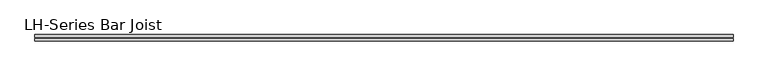
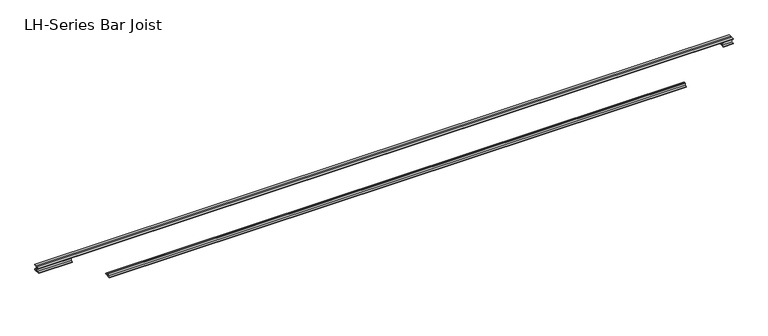
"""IFC4 building model written with IfcOpenShell, lengths in millimetres: beam geometry, LH-Series Bar Joist : 32LH-SP5."""

from ifc_helpers import new_model, si_unit, frame, origin, place, context, project, spatial, polyline, outline, extrude, source, transform, mapped, element, save


def lh_series_bar_joist_ab931e5b(model_context):
    return source(origin(), model_context, "Body", "SweptSolid", [
        extrude(outline(polyline([(12.7, 406.4), (76.2, 406.4), (76.2, 393.7), (25.4, 393.7), (25.4, 342.9), (12.7, 342.9), (12.7, 406.4)])), frame((-8381.9219944, 0.0, 0.0), z_axis=(1.0, 0.0, 0.0), x_axis=(0.0, 1.0, 0.0)), (0.0, 0.0, 1.0), 16208.2969944),
        extrude(outline(polyline([(-12.7, 406.4), (-12.7, 342.9), (-25.4, 342.9), (-25.4, 393.7), (-76.2, 393.7), (-76.2, 406.4), (-12.7, 406.4)])), frame((-8381.9219944, 0.0, 0.0), z_axis=(1.0, 0.0, 0.0), x_axis=(0.0, 1.0, 0.0)), (0.0, 0.0, 1.0), 16208.2969944),
        extrude(outline(polyline([(12.7, -406.4), (12.7, -342.9), (25.4, -342.9), (25.4, -393.7), (76.2, -393.7), (76.2, -406.4), (12.7, -406.4)])), frame((-6734.175, 0.0, 0.0), z_axis=(1.0, 0.0, 0.0), x_axis=(0.0, 1.0, 0.0)), (0.0, 0.0, 1.0), 13468.35),
        extrude(outline(polyline([(-12.7, -406.4), (-76.2, -406.4), (-76.2, -393.7), (-25.4, -393.7), (-25.4, -342.9), (-12.7, -342.9), (-12.7, -406.4)])), frame((-6734.175, 0.0, 0.0), z_axis=(1.0, 0.0, 0.0), x_axis=(0.0, 1.0, 0.0)), (0.0, 0.0, 1.0), 13468.35),
        extrude(outline(polyline([(12.7, 279.4), (12.7, 342.9), (25.4, 342.9), (25.4, 292.1), (76.2, 292.1), (76.2, 279.4), (12.7, 279.4)])), frame((7597.775, 0.0, 0.0), z_axis=(1.0, 0.0, 0.0), x_axis=(0.0, 1.0, 0.0)), (0.0, 0.0, 1.0), 228.6),
        extrude(outline(polyline([(-12.7, 279.4), (-76.2, 279.4), (-76.2, 292.1), (-25.4, 292.1), (-25.4, 342.9), (-12.7, 342.9), (-12.7, 279.4)])), frame((7597.775, 0.0, 0.0), z_axis=(1.0, 0.0, 0.0), x_axis=(0.0, 1.0, 0.0)), (0.0, 0.0, 1.0), 228.6),
        extrude(outline(polyline([(-12.7, 279.4), (-76.2, 279.4), (-76.2, 292.1), (-25.4, 292.1), (-25.4, 342.9), (-12.7, 342.9), (-12.7, 279.4)])), frame((-8381.9219944, 0.0, 0.0), z_axis=(1.0, 0.0, 0.0), x_axis=(0.0, 1.0, 0.0)), (0.0, 0.0, 1.0), 784.1469944),
        extrude(outline(polyline([(76.2, 279.4), (12.7, 279.4), (12.7, 342.9), (25.4, 342.9), (25.4, 292.1), (76.2, 292.1), (76.2, 279.4)])), frame((-8381.9219944, 0.0, 0.0), z_axis=(1.0, 0.0, 0.0), x_axis=(0.0, 1.0, 0.0)), (0.0, 0.0, 1.0), 784.1469944),
    ])


if __name__ == "__main__":
    model = new_model("IFC4")
    model_context = context("Model", 3, world=origin())
    ifc_project = project(units=[si_unit("LENGTHUNIT", "METRE", prefix="MILLI")], contexts=[model_context])
    site = spatial("IfcSite", under=ifc_project)
    building = spatial("IfcBuilding", under=site)
    placement = place(None, origin())
    lh_series_bar_joist_shape = lh_series_bar_joist_ab931e5b(model_context)
    element("IfcBeam", 1, ObjectType="LH-Series Bar Joist : 32LH-SP5", at=placement, inside=building, context=model_context, shape_type="MappedRepresentation", body=[
        mapped(lh_series_bar_joist_shape, transform((0.0, 0.0, 0.0), x_axis=(1.0, 0.0, 0.0), y_axis=(0.0, 1.0, 0.0), z_axis=(0.0, 0.0, 1.0))),
    ])
    save(model, "model.ifc")

# Revit data of these elements
# Type "LH-Series Bar Joist : 32LH-SP5"
#   Assembly Code = "B1010350"
#   Wt = 30
#   Web Thickness = 0' - 1"
#   Variable Panel [instance default] = 5' - 4"
#   Start Offset [instance default] = 0' - 0"
#   Start Extension [instance default] = 0' - 0"
#   Seat Length = 0' - 6"
#   Seat Depth = 0' - 5"
#   IntPanelWidth [instance default] = 5' - 4"
#   IntPanelArrayLength [instance default] = 21' - 4"
#   PanelAreaLength [instance default] = 32' - 0"
#   End Panel = 4' - 0"
#   End Offset [instance default] = 0' - 0"
#   End Extension [instance default] = 0' - 0"
#   Cord Leg = 0' - 2 1/2"
#   Chord Thickness = 0' - 0 1/2"
#   Length [instance default] = 40' - 0"
#   Depth = 2' - 8"
#   Vertical Member Visibility = yes
#   IntPanelArrayNum [instance default] = 4
#   Structural Material = none
# Element 1 (IfcBeam, "LH-Series Bar Joist : 32LH-SP5")
#   Variable Panel = 5' - 5 1/8"
#   Start Extension = 2' - 0.87193"
#   IntPanelArrayLength = 32' - 0"
#   PanelAreaLength = 42' - 10 1/4"
#   End Extension = 0' - 3"
#   Length = 50' - 10 1/4"
#   IntPanelArrayNum = 6
